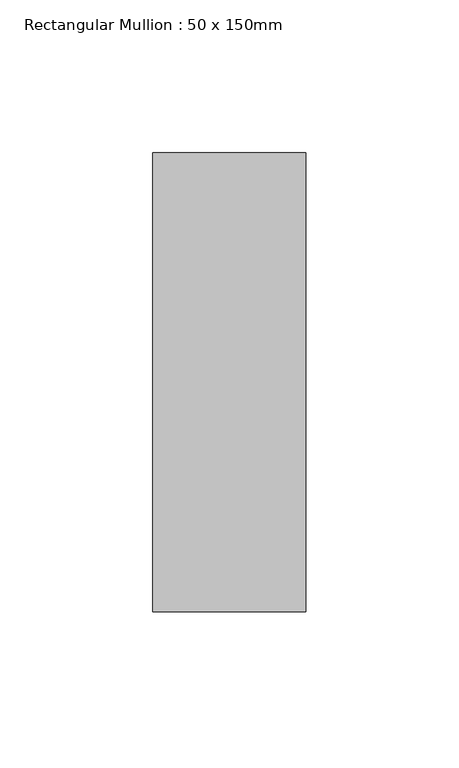
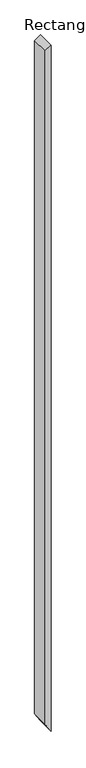
"""IFC4 building model written with IfcOpenShell, lengths in millimetres: member geometry, Rectangular Mullion : 50 x 150mm."""

from ifc_helpers import new_model, si_unit, frame, origin, place, context, project, spatial, polyline, outline, extrude, source, transform, mapped, element, save


def rectangular_mullion_50_x_150mm_abaa279f(model_context):
    return source(origin(), model_context, "Body", "SweptSolid", [
        extrude(outline(polyline([(0.0, 0.0), (-31.871605, -50.0), (-5936.5760489, -50.0), (-6015.015776, 0.0), (0.0, 0.0)])), frame((0.0, -75.0, 0.0), z_axis=(0.0, 1.0, 0.0), x_axis=(0.0, 0.0, 1.0)), (0.0, 0.0, 1.0), 150.0),
    ])


if __name__ == "__main__":
    model = new_model("IFC4")
    model_context = context("Model", 3, world=origin())
    ifc_project = project(units=[si_unit("LENGTHUNIT", "METRE", prefix="MILLI")], contexts=[model_context])
    site = spatial("IfcSite", under=ifc_project)
    building = spatial("IfcBuilding", under=site)
    placement = place(None, origin())
    rectangular_mullion_50_x_150mm_shape = rectangular_mullion_50_x_150mm_abaa279f(model_context)
    element("IfcMember", 1, ObjectType="Rectangular Mullion : 50 x 150mm", at=placement, inside=building, context=model_context, shape_type="MappedRepresentation", body=[
        mapped(rectangular_mullion_50_x_150mm_shape, transform((0.0, 0.0, 0.0), x_axis=(1.0, 0.0, 0.0), y_axis=(0.0, 1.0, 0.0), z_axis=(0.0, 0.0, 1.0))),
    ])
    save(model, "model.ifc")

# Revit data of these elements
# Type "Rectangular Mullion : 50 x 150mm"
#   built-in parameter 1007304 = 0.492126 (stored number, unit not read)
#   built-in parameter 1007301 = 0.082021 (stored number, unit not read)
#   built-in parameter 1007300 = 0.082021 (stored number, unit not read)
# Element 1 (IfcMember, "Rectangular Mullion : 50 x 150mm")
#   Materials on its faces: "Metal - Aluminium"
# Materials
#   "Metal - Aluminium": class "Metal", colour RGB 247 247 247, transparency 0
